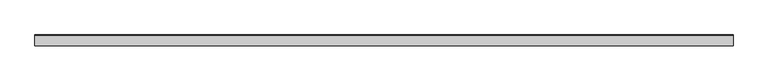
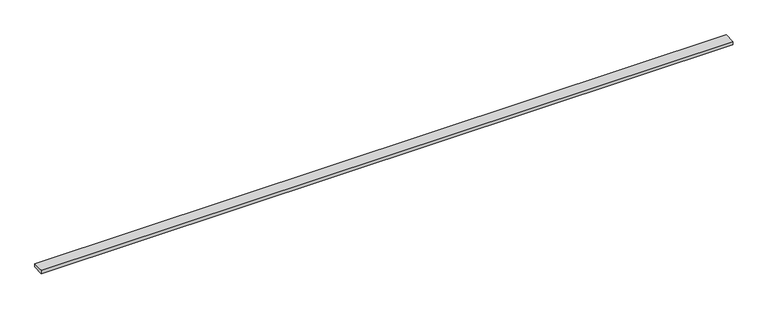
"""IFC4 building model written with IfcOpenShell, lengths in millimetres: proxy geometry, Inner panel:Inner panel:1:Inner panel:1 : Inner panel:Inner panel:300324:2:Inner panel:1:Inner panel:1 : Inner panel:Inner panel:300324:2 : Inner panel:Inner panel:1:Inner panel:1 : Inner panel:Inner panel:300324:300043:50 : Inner panel:Inner panel:1:Inner panel:1 : Inner panel:Inner panel:300324:2:Inner panel:1:Inner panel:1 : Inner panel:Inner panel:300324:2 : Inner panel:Inner panel:1:Inner panel:1 : Inner panel:Inner panel:300324:300043:308120."""

from ifc_helpers import new_model, si_unit, frame, origin, place, context, project, spatial, polyline, outline, extrude, source, transform, mapped, element, save


def generic_models_c5f3da3b(model_context):
    return source(origin(), model_context, "Body", "SweptSolid", [
        extrude(outline(polyline([(0.0, -75.8934963), (0.0, 0.0), (4876.8, 0.0), (4876.8, -75.8934963), (0.0, -75.8934963)])), frame((667264.7367238, -576391.370927, 4033.1979981), z_axis=(0.0, -0.04163054471215047, 0.9991330730923532), x_axis=(-1.0, 0.0, 0.0)), (0.0, 0.0, 1.0), 25.4),
    ])


if __name__ == "__main__":
    model = new_model("IFC4")
    model_context = context("Model", 3, world=origin())
    ifc_project = project(units=[si_unit("LENGTHUNIT", "METRE", prefix="MILLI")], contexts=[model_context])
    site = spatial("IfcSite", under=ifc_project)
    building = spatial("IfcBuilding", under=site)
    placement = place(None, origin())
    generic_models_shape = generic_models_c5f3da3b(model_context)
    element("IfcBuildingElementProxy", 1, Name="Inner panel:Inner panel:1:Inner panel:1 : Inner panel:Inner panel:300324:2:Inner panel:1:Inner panel:1 : Inner panel:Inner panel:300324:2 : Inner panel:Inner panel:1:Inner panel:1 : Inner panel:Inner panel:300324:300043:50 : Inner panel:Inner panel:1:Inner panel:1 : Inner panel:Inner panel:300324:2:Inner panel:1:Inner panel:1 : Inner panel:Inner panel:300324:2 : Inner panel:Inner panel:1:Inner panel:1 : Inner panel:Inner panel:300324:300043:308120", ObjectType="Inner panel:Inner panel:1:Inner panel:1 : Inner panel:Inner panel:300324:2:Inner panel:1:Inner panel:1 : Inner panel:Inner panel:300324:2 : Inner panel:Inner panel:1:Inner panel:1 : Inner panel:Inner panel:300324:300043:50 : Inner panel:Inner panel:1:Inner panel:1 : Inner panel:Inner panel:300324:2:Inner panel:1:Inner panel:1 : Inner panel:Inner panel:300324:2 : Inner panel:Inner panel:1:Inner panel:1 : Inner panel:Inner panel:300324:300043:308120", at=placement, inside=building, context=model_context, shape_type="MappedRepresentation", body=[
        mapped(generic_models_shape, transform((0.0, 0.0, 0.0), x_axis=(1.0, 0.0, 0.0), y_axis=(0.0, 1.0, 0.0), z_axis=(0.0, 0.0, 1.0))),
    ])
    save(model, "model.ifc")

# Revit data of these elements
# Type "Inner panel:Inner panel:1:Inner panel:1 : Inner panel:Inner panel:300324:2:Inner panel:1:Inner panel:1 : Inner panel:Inner panel:300324:2 : Inner panel:Inner panel:1:Inner panel:1 : Inner panel:Inner panel:300324:300043:50 : Inner panel:Inner panel:1:Inner panel:1 : Inner panel:Inner panel:300324:2:Inner panel:1:Inner panel:1 : Inner panel:Inner panel:300324:2 : Inner panel:Inner panel:1:Inner panel:1 : Inner panel:Inner panel:300324:300043:308120"
#   NameOverride = "Inner panel:Inner panel:1:Inner panel:1 : Inner panel:Inner panel:300324:2:Inner panel:1:Inner panel:1 : Inner panel:Inner panel:300324:2 : Inner panel:Inner panel:1:Inner panel:1 : Inner panel:Inner panel:300324:300043:308120"
#   ObjectTypeOverride = "Inner panel:1:Inner panel:1 : Inner panel:Inner panel:300324:2 : Inner panel:Inner panel:1:Inner panel:1 : Inner panel:Inner panel:300324:300043"
#   Reference = "Inner panel"
#   Tag = "308120"
# Element 1 (IfcBuildingElementProxy, "Inner panel:Inner panel:1:Inner panel:1 : Inner panel:Inner panel:300324:2:Inner panel:1:Inner panel:1 : Inner panel:Inner panel:300324:2 : Inner panel:Inner panel:1:Inner panel:1 : Inner panel:Inner panel:300324:300043:50 : Inner panel:Inner panel:1:Inner panel:1 : Inner panel:Inner panel:300324:2:Inner panel:1:Inner panel:1 : Inner panel:Inner panel:300324:2 : Inner panel:Inner panel:1:Inner panel:1 : Inner panel:Inner panel:300324:300043:308120")
#   Materials on its faces: "1\" THERMAL SPACER @ PURLIN"
# Materials
#   "1\" THERMAL SPACER @ PURLIN": class "Unassigned", colour RGB 205 188 106, transparency 0, Cost = 0
